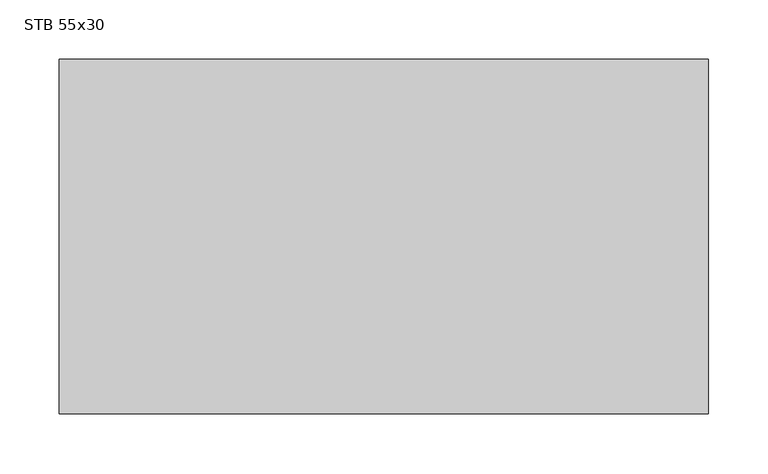
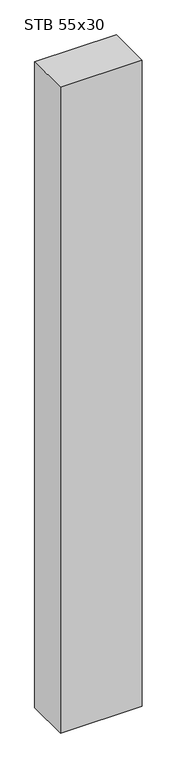
"""IFC4 building model written with IfcOpenShell, lengths in millimetres: column geometry, STB Stütze - rechteckig : STB 55x30."""

import ifcopenshell
import ifcopenshell.guid

model = None  # the IFC model being written
_history = None  # IfcOwnerHistory: only IFC2X3 demands one
_inside = {}  # id of a spatial element -> (the spatial element, [elements in it])
_under = {}  # id of a project, library or spatial element -> (it, [spatial elements below it])
_declared = {}  # id of a project -> (the project, [libraries it declares])
_typed = {}  # id of a type object -> (the type object, [elements of that type])
_made_of = {}  # id of a material, layer set ... -> (it, [elements and type objects made of it])


def new_model(schema):
    """Start an empty IFC model of exactly this schema.

    Asked for "IFC4X3", IfcOpenShell would pick the latest addendum, in which some entities
    have other attributes; the version numbers below select the first issue.
    IFC2X3 requires an IfcOwnerHistory on every rooted entity: one is made here for all.
    """
    global model, _history
    if schema == "IFC4X3":
        model = ifcopenshell.file(schema_version=(4, 3, 0, 0))
    else:
        model = ifcopenshell.file(schema=schema)
    _inside.clear()
    _under.clear()
    _declared.clear()
    _typed.clear()
    _made_of.clear()
    _history = None
    if model.schema == "IFC2X3":
        org = make("IfcOrganization", Name="unknown")
        user = make(
            "IfcPersonAndOrganization",
            ThePerson=make("IfcPerson", FamilyName="unknown"),
            TheOrganization=org,
        )
        app = make(
            "IfcApplication",
            ApplicationDeveloper=org,
            Version="unknown",
            ApplicationFullName="unknown",
            ApplicationIdentifier="unknown",
        )
        _history = make(
            "IfcOwnerHistory",
            OwningUser=user,
            OwningApplication=app,
            ChangeAction="ADDED",
            CreationDate=0,
        )
    return model


def make(cls, **values):
    """One entity of the class cls with the attributes given. An attribute that is None is left unset."""
    return model.create_entity(
        cls, **{name: value for name, value in values.items() if value is not None}
    )


def rooted(cls, **values):
    """An entity with a GlobalId (a new one), such as an element, a storey or a relation."""
    return make(cls, GlobalId=ifcopenshell.guid.new(), OwnerHistory=_history, **values)


def si_unit(unit_type, name, prefix=None):
    """IfcSIUnit, for example si_unit("LENGTHUNIT", "METRE", prefix="MILLI")."""
    return make("IfcSIUnit", UnitType=unit_type, Prefix=prefix, Name=name)


def assignment(units):
    """IfcUnitAssignment: the units of a project."""
    return None if units is None else make("IfcUnitAssignment", Units=units)


def point(xyz):
    """IfcCartesianPoint."""
    return None if xyz is None else make("IfcCartesianPoint", Coordinates=xyz)


def direction(xyz):
    """IfcDirection."""
    return None if xyz is None else make("IfcDirection", DirectionRatios=xyz)


def frame(location, z_axis=None, x_axis=None):
    """IfcAxis2Placement3D, a coordinate frame: its origin and axes. An axis left out is left unset."""
    return make(
        "IfcAxis2Placement3D",
        Location=point(location),
        Axis=direction(z_axis),
        RefDirection=direction(x_axis),
    )


def origin():
    """The frame at (0, 0, 0) with its axes left unset."""
    return frame((0.0, 0.0, 0.0))


def place(relative_to, where):
    """IfcLocalPlacement: puts the frame where relative to a parent placement (None: the world)."""
    return make(
        "IfcLocalPlacement", PlacementRelTo=relative_to, RelativePlacement=where
    )


def context(
    kind, dimensions, precision=None, world=None, true_north=None, identifier=None
):
    """IfcGeometricRepresentationContext, for example the 3D "Model" context."""
    return make(
        "IfcGeometricRepresentationContext",
        ContextIdentifier=identifier,
        ContextType=kind,
        CoordinateSpaceDimension=dimensions,
        Precision=precision,
        WorldCoordinateSystem=world,
        TrueNorth=true_north,
    )


def project(units=None, contexts=None):
    """IfcProject with its units and contexts."""
    return rooted(
        "IfcProject",
        Name="project",
        RepresentationContexts=contexts,
        UnitsInContext=assignment(units),
    )


def spatial(cls, under=None, at=None, **own):
    """A site, building, storey or space (cls), placed at a placement, below another one or the project."""
    s = rooted(cls, ObjectPlacement=at, **own)
    if under is not None:
        _under.setdefault(under.id(), (under, []))[1].append(s)
    return s


def polyline(points):
    """IfcPolyline through the points."""
    return make("IfcPolyline", Points=[point(p) for p in points])


def outline(outer, holes=None, kind="AREA"):
    """IfcArbitraryClosedProfileDef: a profile drawn as a closed curve; with holes, ...WithVoids."""
    if holes is None:
        return make("IfcArbitraryClosedProfileDef", ProfileType=kind, OuterCurve=outer)
    return make(
        "IfcArbitraryProfileDefWithVoids",
        ProfileType=kind,
        OuterCurve=outer,
        InnerCurves=holes,
    )


def extrude(swept, where, along, depth):
    """IfcExtrudedAreaSolid: the profile swept, set in the frame where, extruded along a direction by depth."""
    return make(
        "IfcExtrudedAreaSolid",
        SweptArea=swept,
        Position=where,
        ExtrudedDirection=direction(along),
        Depth=depth,
    )


def shape(context_of_items, identifier, shape_type, items):
    """IfcShapeRepresentation: the items that make up one representation, for example the "Body"."""
    return make(
        "IfcShapeRepresentation",
        ContextOfItems=context_of_items,
        RepresentationIdentifier=identifier,
        RepresentationType=shape_type,
        Items=items,
    )


def source(mapping_origin, context_of_items, identifier, shape_type, items):
    """IfcRepresentationMap: a shape defined once, which mapped items show again and again."""
    return make(
        "IfcRepresentationMap",
        MappingOrigin=mapping_origin,
        MappedRepresentation=shape(context_of_items, identifier, shape_type, items),
    )


def transform(
    local_origin,
    x_axis=None,
    y_axis=None,
    z_axis=None,
    scale=None,
    scale2=None,
    scale3=None,
    uniform=True,
):
    """IfcCartesianTransformationOperator3D, or its non-uniform kind. x_axis, y_axis, z_axis: its Axis1, 2, 3."""
    if uniform:
        return make(
            "IfcCartesianTransformationOperator3D",
            Axis1=direction(x_axis),
            Axis2=direction(y_axis),
            LocalOrigin=point(local_origin),
            Scale=scale,
            Axis3=direction(z_axis),
        )
    return make(
        "IfcCartesianTransformationOperator3DnonUniform",
        Axis1=direction(x_axis),
        Axis2=direction(y_axis),
        LocalOrigin=point(local_origin),
        Scale=scale,
        Axis3=direction(z_axis),
        Scale2=scale2,
        Scale3=scale3,
    )


def mapped(mapping_source, mapping_target):
    """IfcMappedItem: shows the shape of a source again, moved by a transform."""
    return make(
        "IfcMappedItem", MappingSource=mapping_source, MappingTarget=mapping_target
    )


def made_of(thing, what):
    """Note that an element or type object is made of a material, layer set ...; save() writes the relation."""
    if what is not None:
        _made_of.setdefault(what.id(), (what, []))[1].append(thing)
    return thing


def element(
    cls,
    number,
    at=None,
    inside=None,
    cuts=None,
    type_object=None,
    material=None,
    context=None,
    identifier="Body",
    shape_type=None,
    held_by="IfcProductDefinitionShape",
    body=None,
    shapes=None,
    **own,
):
    """One element of the class cls, such as IfcWall. Its Tag is "e" and its number.

    at: its placement. inside: the storey or other place that contains it. cuts: it is an
    opening in that element (IfcRelVoidsElement). A single representation is given by context,
    identifier, shape_type and body (its items); several are given by shapes. held_by: the class
    of the entity that holds the representations. save() writes the other relations.
    """
    e = rooted(cls, Tag="e%d" % number, ObjectPlacement=at, **own)
    if body is not None:
        shapes = [shape(context, identifier, shape_type, body)]
    if shapes is not None:
        e.Representation = make(held_by, Representations=shapes)
    if inside is not None:
        _inside.setdefault(inside.id(), (inside, []))[1].append(e)
    if cuts is not None:
        rooted(
            "IfcRelVoidsElement", RelatingBuildingElement=cuts, RelatedOpeningElement=e
        )
    if type_object is not None:
        _typed.setdefault(type_object.id(), (type_object, []))[1].append(e)
    return made_of(e, material)


def aggregate(whole, parts):
    """IfcRelAggregates: a whole, such as a stair, and the parts it consists of."""
    return rooted("IfcRelAggregates", RelatingObject=whole, RelatedObjects=parts)


def save(model, path):
    """Write the relations noted so far, then the file.

    IfcRelAggregates (storeys below a building ...), IfcRelContainedInSpatialStructure (elements
    in a storey), IfcRelDefinesByType, IfcRelAssociatesMaterial and IfcRelDeclares: one each for
    every whole, place, type object, material and project.
    """
    for whole, parts in _under.values():
        aggregate(whole, parts)
    for where, things in _inside.values():
        rooted(
            "IfcRelContainedInSpatialStructure",
            RelatedElements=things,
            RelatingStructure=where,
        )
    for kind, things in _typed.values():
        rooted("IfcRelDefinesByType", RelatedObjects=things, RelatingType=kind)
    for what, things in _made_of.values():
        rooted("IfcRelAssociatesMaterial", RelatedObjects=things, RelatingMaterial=what)
    for by, libraries in _declared.values():
        rooted("IfcRelDeclares", RelatingContext=by, RelatedDefinitions=libraries)
    model.write(path)


def stb_55x30_396f348b(model_context):
    return source(origin(), model_context, "Body", "SweptSolid", [
        extrude(outline(polyline([(275.0, 150.0), (275.0, -150.0), (-275.0, -150.0), (-275.0, 150.0), (275.0, 150.0)])), frame((0.0, 0.0, -1580.0), z_axis=(0.0, 0.0, 1.0), x_axis=(1.0, 0.0, 0.0)), (0.0, 0.0, 1.0), 4600.0),
    ])


if __name__ == "__main__":
    model = new_model("IFC4")
    model_context = context("Model", 3, world=origin())
    ifc_project = project(units=[si_unit("LENGTHUNIT", "METRE", prefix="MILLI")], contexts=[model_context])
    site = spatial("IfcSite", under=ifc_project)
    building = spatial("IfcBuilding", under=site)
    placement = place(None, origin())
    stb_55x30_shape = stb_55x30_396f348b(model_context)
    element("IfcColumn", 1, ObjectType="STB Stütze - rechteckig : STB 55x30", at=placement, inside=building, context=model_context, shape_type="MappedRepresentation", body=[
        mapped(stb_55x30_shape, transform((0.0, 0.0, 0.0), x_axis=(1.0, 0.0, 0.0), y_axis=(0.0, 1.0, 0.0), z_axis=(0.0, 0.0, 1.0))),
    ])
    save(model, "model.ifc")

# Revit data of these elements
# Type "STB Stütze - rechteckig : STB 55x30"
#   Breite = 0.550 m
#   Tiefe = 0.300 m
#   Structural Material [instance default] = Stahlbeton - Ortbeton
# Element 1 (IfcColumn, "STB Stütze - rechteckig : STB 55x30")
#   Materials on its faces: "Stahlbeton - Ortbeton"
# Materials
#   "Stahlbeton - Ortbeton": class "Beton", colour RGB 247 247 247, transparency 0, Cost = 0
